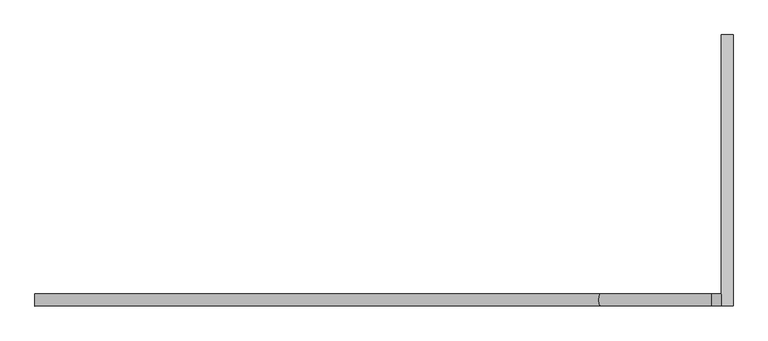
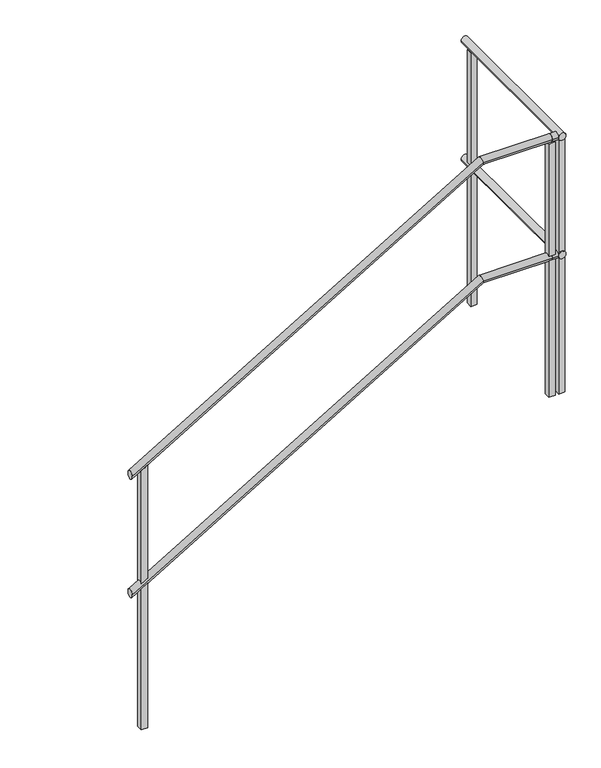
"""IFC4 building model written with IfcOpenShell, lengths in millimetres: railing geometry."""

from ifc_helpers import new_model, si_unit, frame, origin, place, context, project, spatial, polyline, circle_curve, ellipse_curve, outline, extrude, source, transform, mapped, element, save
from ifc_brep_helpers import plane_surface, cylinder_surface, advanced_brep


def railing_e31db196(model_context):
    return source(origin(), model_context, "Body", "SolidModel", [
        advanced_brep(
        [(35195.0, 4.9208589, 749.1723166), (35195.0, -25.0791411, 749.1723166), (36599.1264386, 4.9208589, 1584.9618634), (36599.1264386, -25.0791411, 1584.9618634), (36875.0, 4.9208589, 1584.9618634), (36875.0, -25.0791411, 1584.9618634)],
        [
            (0, 1, ellipse_curve(frame((35195.0, -10.0791411, 749.1723166), z_axis=(-1.0, 0.0, 0.0), x_axis=(0.0, 0.0, -1.0)), 17.4562134, 15.0)),
            (1, 0, ellipse_curve(frame((35195.0, -10.0791411, 749.1723166), z_axis=(-1.0, 0.0, 0.0), x_axis=(0.0, 0.0, -1.0)), 17.4562134, 15.0)),
            (0, 2),
            (2, 3, ellipse_curve(frame((36599.1264386, -10.0791411, 1584.9618634), z_axis=(-0.9641817474962143, 0.0, -0.2652424509673111), x_axis=(0.265242450967311, 0.0, -0.9641817474962144)), 15.5572329, 15.0)),
            (3, 1),
            (3, 2, ellipse_curve(frame((36599.1264386, -10.0791411, 1584.9618634), z_axis=(-0.9641817474962143, 0.0, -0.2652424509673111), x_axis=(0.265242450967311, 0.0, -0.9641817474962144)), 15.5572329, 15.0)),
            (4, 5, circle_curve(frame((36875.0, -10.0791411, 1584.9618634), z_axis=(1.0, 0.0, 0.0), x_axis=(0.0, -1.0, 0.0)), 15.0)),
            (5, 4, circle_curve(frame((36875.0, -10.0791411, 1584.9618634), z_axis=(1.0, 0.0, 0.0), x_axis=(0.0, -1.0, 0.0)), 15.0)),
            (2, 4),
            (5, 3),
        ],
        [
            plane_surface(frame((35195.0, -10.0791411, 766.62853), z_axis=(-1.0, 0.0, 0.0), x_axis=(0.0, 1.0, 0.0))),
            cylinder_surface(frame((35202.6722579, -10.0791411, 753.7391368), z_axis=(-0.8592928844097072, 0.0, -0.5114838597676818), x_axis=(0.0, -1.0, 0.0)), 15.0),
            plane_surface(frame((36875.0, -10.0791411, 1599.9618634), z_axis=(1.0, 0.0, 0.0), x_axis=(0.0, 1.0, 0.0))),
            cylinder_surface(frame((36595.0, -10.0791411, 1584.9618634), z_axis=(-1.0, 0.0, 0.0), x_axis=(0.0, -1.0, 0.0)), 15.0),
        ],
        [
            (0, [[1, 2]]),
            (1, [[-1, 3, 4, 5]]),
            (1, [[-2, -5, 6, -3]]),
            (2, [[7, 8]]),
            (3, [[-4, 9, -8, 10]]),
            (3, [[-6, -10, -7, -9]]),
        ],
    ),
        advanced_brep(
        [(36875.0, 4.9208589, 1584.9618634), (36875.0, -25.0791411, 1584.9618634), (36899.6, 4.9208589, 1584.9618634), (36899.6, -25.0791411, 1584.9618634)],
        [
            (0, 1, circle_curve(frame((36875.0, -10.0791411, 1584.9618634), z_axis=(-1.0, 0.0, 0.0), x_axis=(0.0, -1.0, 0.0)), 15.0)),
            (1, 0, circle_curve(frame((36875.0, -10.0791411, 1584.9618634), z_axis=(-1.0, 0.0, 0.0), x_axis=(0.0, -1.0, 0.0)), 15.0)),
            (2, 3, circle_curve(frame((36899.6, -10.0791411, 1584.9618634), z_axis=(1.0, 0.0, 0.0), x_axis=(0.0, -1.0, 0.0)), 15.0)),
            (3, 2, circle_curve(frame((36899.6, -10.0791411, 1584.9618634), z_axis=(1.0, 0.0, 0.0), x_axis=(0.0, -1.0, 0.0)), 15.0)),
            (0, 2),
            (3, 1),
        ],
        [
            plane_surface(frame((36875.0, -10.0791411, 1599.9618634), z_axis=(-1.0, 0.0, 0.0), x_axis=(0.0, 1.0, 0.0))),
            plane_surface(frame((36899.6, -10.0791411, 1599.9618634), z_axis=(1.0, 0.0, 0.0), x_axis=(0.0, 1.0, 0.0))),
            cylinder_surface(frame((36875.0, -10.0791411, 1584.9618634), z_axis=(-1.0, 0.0, 0.0), x_axis=(0.0, -1.0, 0.0)), 15.0),
        ],
        [
            (0, [[1, 2]]),
            (1, [[3, 4]]),
            (2, [[-1, 5, -4, 6]]),
            (2, [[-2, -6, -3, -5]]),
        ],
    ),
        advanced_brep(
        [(36899.6, -25.0791411, 1584.9618634), (36929.6, -25.0791411, 1584.9618634), (36899.6, 649.5208589, 1584.9618634), (36929.6, 649.5208589, 1584.9618634)],
        [
            (0, 1, circle_curve(frame((36914.6, -25.0791411, 1584.9618634), z_axis=(0.0, -1.0, 0.0), x_axis=(1.0, 0.0, 0.0)), 15.0)),
            (1, 0, circle_curve(frame((36914.6, -25.0791411, 1584.9618634), z_axis=(0.0, -1.0, 0.0), x_axis=(1.0, 0.0, 0.0)), 15.0)),
            (2, 3, circle_curve(frame((36914.6, 649.5208589, 1584.9618634), z_axis=(0.0, 1.0, 0.0), x_axis=(1.0, 0.0, 0.0)), 15.0)),
            (3, 2, circle_curve(frame((36914.6, 649.5208589, 1584.9618634), z_axis=(0.0, 1.0, 0.0), x_axis=(1.0, 0.0, 0.0)), 15.0)),
            (0, 2),
            (3, 1),
        ],
        [
            plane_surface(frame((36914.6, -25.0791411, 1599.9618634), z_axis=(0.0, -1.0, 0.0), x_axis=(0.0, 0.0, 1.0))),
            plane_surface(frame((36914.6, 649.5208589, 1599.9618634), z_axis=(0.0, 1.0, 0.0), x_axis=(0.0, 0.0, 1.0))),
            cylinder_surface(frame((36914.6, -25.0791411, 1584.9618634), z_axis=(0.0, -1.0, 0.0), x_axis=(1.0, 0.0, 0.0)), 15.0),
        ],
        [
            (0, [[1, 2]]),
            (1, [[3, 4]]),
            (2, [[-1, 5, -4, 6]]),
            (2, [[-2, -6, -3, -5]]),
        ],
    ),
        advanced_brep(
        [(35195.0, 4.9208589, 1249.1723166), (35195.0, -25.0791411, 1249.1723166), (36599.1264386, 4.9208589, 2084.9618634), (36599.1264386, -25.0791411, 2084.9618634), (36875.0, 4.9208589, 2084.9618634), (36875.0, -25.0791411, 2084.9618634)],
        [
            (0, 1, ellipse_curve(frame((35195.0, -10.0791411, 1249.1723166), z_axis=(-1.0, 0.0, 0.0), x_axis=(0.0, 0.0, -1.0)), 17.4562134, 15.0)),
            (1, 0, ellipse_curve(frame((35195.0, -10.0791411, 1249.1723166), z_axis=(-1.0, 0.0, 0.0), x_axis=(0.0, 0.0, -1.0)), 17.4562134, 15.0)),
            (0, 2),
            (2, 3, ellipse_curve(frame((36599.1264386, -10.0791411, 2084.9618634), z_axis=(-0.9641817474962143, 0.0, -0.2652424509673111), x_axis=(0.265242450967311, 0.0, -0.9641817474962144)), 15.5572329, 15.0)),
            (3, 1),
            (3, 2, ellipse_curve(frame((36599.1264386, -10.0791411, 2084.9618634), z_axis=(-0.9641817474962143, 0.0, -0.2652424509673111), x_axis=(0.265242450967311, 0.0, -0.9641817474962144)), 15.5572329, 15.0)),
            (4, 5, circle_curve(frame((36875.0, -10.0791411, 2084.9618634), z_axis=(1.0, 0.0, 0.0), x_axis=(0.0, -1.0, 0.0)), 15.0)),
            (5, 4, circle_curve(frame((36875.0, -10.0791411, 2084.9618634), z_axis=(1.0, 0.0, 0.0), x_axis=(0.0, -1.0, 0.0)), 15.0)),
            (2, 4),
            (5, 3),
        ],
        [
            plane_surface(frame((35195.0, -10.0791411, 1266.62853), z_axis=(-1.0, 0.0, 0.0), x_axis=(0.0, 1.0, 0.0))),
            cylinder_surface(frame((35202.6722579, -10.0791411, 1253.7391368), z_axis=(-0.8592928844097072, 0.0, -0.5114838597676818), x_axis=(0.0, -1.0, 0.0)), 15.0),
            plane_surface(frame((36875.0, -10.0791411, 2099.9618634), z_axis=(1.0, 0.0, 0.0), x_axis=(0.0, 1.0, 0.0))),
            cylinder_surface(frame((36595.0, -10.0791411, 2084.9618634), z_axis=(-1.0, 0.0, 0.0), x_axis=(0.0, -1.0, 0.0)), 15.0),
        ],
        [
            (0, [[1, 2]]),
            (1, [[-1, 3, 4, 5]]),
            (1, [[-2, -5, 6, -3]]),
            (2, [[7, 8]]),
            (3, [[-4, 9, -8, 10]]),
            (3, [[-6, -10, -7, -9]]),
        ],
    ),
        advanced_brep(
        [(36875.0, 4.9208589, 2084.9618634), (36875.0, -25.0791411, 2084.9618634), (36899.6, 4.9208589, 2084.9618634), (36899.6, -25.0791411, 2084.9618634)],
        [
            (0, 1, circle_curve(frame((36875.0, -10.0791411, 2084.9618634), z_axis=(-1.0, 0.0, 0.0), x_axis=(0.0, -1.0, 0.0)), 15.0)),
            (1, 0, circle_curve(frame((36875.0, -10.0791411, 2084.9618634), z_axis=(-1.0, 0.0, 0.0), x_axis=(0.0, -1.0, 0.0)), 15.0)),
            (2, 3, circle_curve(frame((36899.6, -10.0791411, 2084.9618634), z_axis=(1.0, 0.0, 0.0), x_axis=(0.0, -1.0, 0.0)), 15.0)),
            (3, 2, circle_curve(frame((36899.6, -10.0791411, 2084.9618634), z_axis=(1.0, 0.0, 0.0), x_axis=(0.0, -1.0, 0.0)), 15.0)),
            (0, 2),
            (3, 1),
        ],
        [
            plane_surface(frame((36875.0, -10.0791411, 2099.9618634), z_axis=(-1.0, 0.0, 0.0), x_axis=(0.0, 1.0, 0.0))),
            plane_surface(frame((36899.6, -10.0791411, 2099.9618634), z_axis=(1.0, 0.0, 0.0), x_axis=(0.0, 1.0, 0.0))),
            cylinder_surface(frame((36875.0, -10.0791411, 2084.9618634), z_axis=(-1.0, 0.0, 0.0), x_axis=(0.0, -1.0, 0.0)), 15.0),
        ],
        [
            (0, [[1, 2]]),
            (1, [[3, 4]]),
            (2, [[-1, 5, -4, 6]]),
            (2, [[-2, -6, -3, -5]]),
        ],
    ),
        advanced_brep(
        [(36899.6, -25.0791411, 2084.9618634), (36929.6, -25.0791411, 2084.9618634), (36899.6, 649.5208589, 2084.9618634), (36929.6, 649.5208589, 2084.9618634)],
        [
            (0, 1, circle_curve(frame((36914.6, -25.0791411, 2084.9618634), z_axis=(0.0, -1.0, 0.0), x_axis=(1.0, 0.0, 0.0)), 15.0)),
            (1, 0, circle_curve(frame((36914.6, -25.0791411, 2084.9618634), z_axis=(0.0, -1.0, 0.0), x_axis=(1.0, 0.0, 0.0)), 15.0)),
            (2, 3, circle_curve(frame((36914.6, 649.5208589, 2084.9618634), z_axis=(0.0, 1.0, 0.0), x_axis=(1.0, 0.0, 0.0)), 15.0)),
            (3, 2, circle_curve(frame((36914.6, 649.5208589, 2084.9618634), z_axis=(0.0, 1.0, 0.0), x_axis=(1.0, 0.0, 0.0)), 15.0)),
            (0, 2),
            (3, 1),
        ],
        [
            plane_surface(frame((36914.6, -25.0791411, 2099.9618634), z_axis=(0.0, -1.0, 0.0), x_axis=(0.0, 0.0, 1.0))),
            plane_surface(frame((36914.6, 649.5208589, 2099.9618634), z_axis=(0.0, 1.0, 0.0), x_axis=(0.0, 0.0, 1.0))),
            cylinder_surface(frame((36914.6, -25.0791411, 2084.9618634), z_axis=(0.0, -1.0, 0.0), x_axis=(1.0, 0.0, 0.0)), 15.0),
        ],
        [
            (0, [[1, 2]]),
            (1, [[3, 4]]),
            (2, [[-1, 5, -4, 6]]),
            (2, [[-2, -6, -3, -5]]),
        ],
    ),
        extrude(outline(polyline([(36902.1, -22.5791411), (36902.1, 2.4208589), (36927.1, 2.4208589), (36927.1, -22.5791411), (36902.1, -22.5791411)])), frame((0.0, 0.0, 999.9618634), z_axis=(0.0, 0.0, 1.0), x_axis=(1.0, 0.0, 0.0)), (0.0, 0.0, 1.0), 1070.0),
        extrude(outline(polyline([(36862.5, -22.5791411), (36862.5, 2.4208589), (36887.5, 2.4208589), (36887.5, -22.5791411), (36862.5, -22.5791411)])), frame((0.0, 0.0, 999.9618634), z_axis=(0.0, 0.0, 1.0), x_axis=(1.0, 0.0, 0.0)), (0.0, 0.0, 1.0), 1070.0),
        extrude(outline(polyline([(36927.1, 587.0208589), (36902.1, 587.0208589), (36902.1, 612.0208589), (36927.1, 612.0208589), (36927.1, 587.0208589)])), frame((0.0, 0.0, 999.9618634), z_axis=(0.0, 0.0, 1.0), x_axis=(1.0, 0.0, 0.0)), (0.0, 0.0, 1.0), 1070.0),
        extrude(outline(polyline([(1258.9499586, 35232.5), (166.62853, 35232.5), (166.62853, 35257.5), (1273.830911, 35257.5), (1258.9499586, 35232.5)])), frame((0.0, -22.5791411, 0.0), z_axis=(0.0, 1.0, 0.0), x_axis=(0.0, 0.0, 1.0)), (0.0, 0.0, 1.0), 25.0),
    ])


if __name__ == "__main__":
    model = new_model("IFC4")
    model_context = context("Model", 3, world=origin())
    ifc_project = project(units=[si_unit("LENGTHUNIT", "METRE", prefix="MILLI")], contexts=[model_context])
    site = spatial("IfcSite", under=ifc_project)
    building = spatial("IfcBuilding", under=site)
    placement = place(None, origin())
    railing_shape = railing_e31db196(model_context)
    element("IfcRailing", 1, at=placement, inside=building, context=model_context, shape_type="MappedRepresentation", body=[
        mapped(railing_shape, transform((0.0, 0.0, 0.0), x_axis=(1.0, 0.0, 0.0), y_axis=(0.0, 1.0, 0.0), z_axis=(0.0, 0.0, 1.0))),
    ])
    save(model, "model.ifc")
